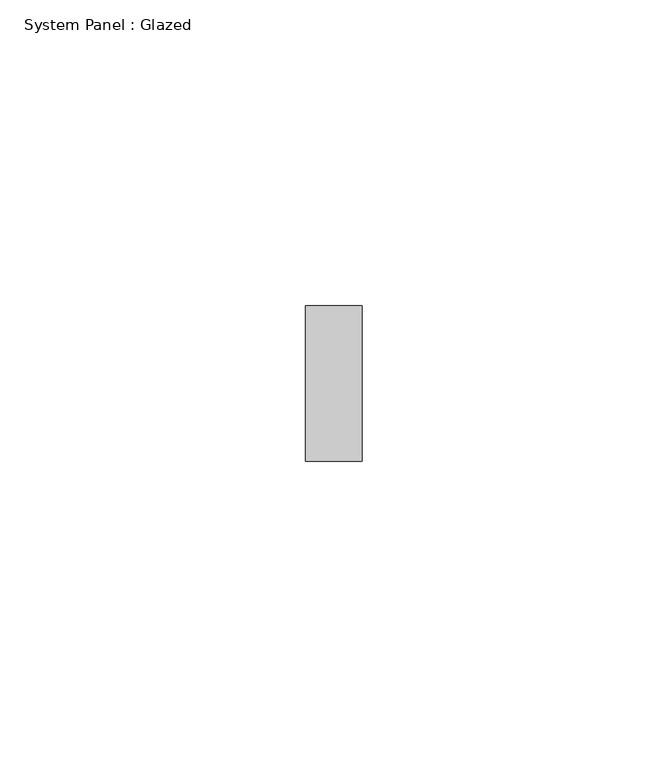
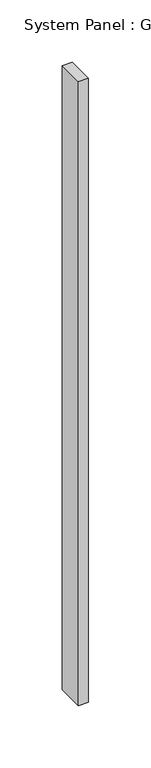
"""IFC4 building model written with IfcOpenShell, lengths in millimetres: plate geometry, System Panel : Glazed."""

from ifc_helpers import new_model, si_unit, origin, origin_with_axes, place, context, project, spatial, polyline, outline, extrude, source, transform, mapped, element, save


def system_panel_glazed_b8323001(model_context):
    return source(origin(), model_context, "Body", "SweptSolid", [
        extrude(outline(polyline([(4.6013366, 19.05), (-4.6013366, 19.05), (-4.6013366, 44.45), (4.6013366, 44.45), (4.6013366, 19.05)])), origin_with_axes(), (0.0, 0.0, 1.0), 609.6),
    ])


if __name__ == "__main__":
    model = new_model("IFC4")
    model_context = context("Model", 3, world=origin())
    ifc_project = project(units=[si_unit("LENGTHUNIT", "METRE", prefix="MILLI")], contexts=[model_context])
    site = spatial("IfcSite", under=ifc_project)
    building = spatial("IfcBuilding", under=site)
    placement = place(None, origin())
    system_panel_glazed_shape = system_panel_glazed_b8323001(model_context)
    element("IfcPlate", 1, ObjectType="System Panel : Glazed", at=placement, inside=building, context=model_context, shape_type="MappedRepresentation", body=[
        mapped(system_panel_glazed_shape, transform((0.0, 0.0, 0.0), x_axis=(1.0, 0.0, 0.0), y_axis=(0.0, 1.0, 0.0), z_axis=(0.0, 0.0, 1.0))),
    ])
    save(model, "model.ifc")

# Revit data of these elements
# Element 1 (IfcPlate, "System Panel : Glazed")
#   Materials on its faces: "Glass"
# Materials
#   "Glass": class "Glass", colour RGB 0 128 192, transparency 0.75
